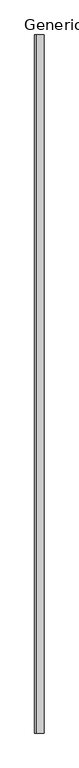
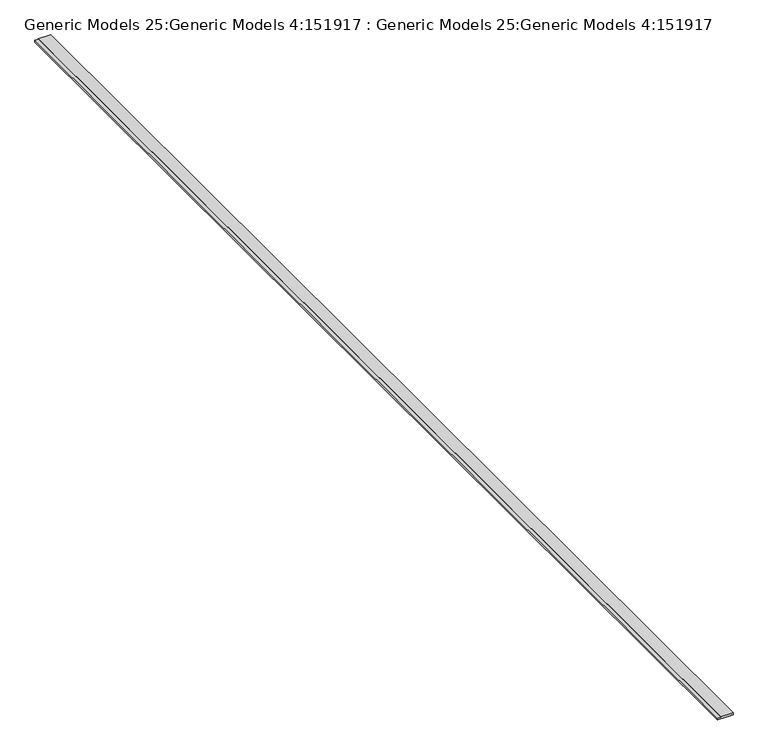
"""IFC4 building model written with IfcOpenShell, lengths in millimetres: proxy geometry, Generic Models 25:Generic Models 4:151917 : Generic Models 25:Generic Models 4:151917."""

from ifc_helpers import new_model, si_unit, frame, origin, place, context, project, spatial, polyline, outline, extrude, source, transform, mapped, element, save


def generic_models_25_generic_models_4_151917_generic_models_25_53bbe27b(model_context):
    return source(origin(), model_context, "Body", "SweptSolid", [
        extrude(outline(polyline([(3046.095, 8497.8650291), (3046.095, 8520.308213), (3067.05, 8520.308213), (3067.05, 8390.926963), (3065.78, 8390.926963), (3065.78, 8354.096963), (3046.095, 8354.096963), (3046.095, 8356.306763), (3047.8274564, 8356.306763), (3047.8274564, 8357.576763), (3044.825, 8357.576763), (3044.825, 8497.8650291), (3046.095, 8497.8650291)])), frame((0.0, -477.1974793, 0.0), z_axis=(0.0, 1.0, 0.0), x_axis=(0.0, 0.0, 1.0)), (0.0, 0.0, 1.0), 12446.0),
    ])


if __name__ == "__main__":
    model = new_model("IFC4")
    model_context = context("Model", 3, world=origin())
    ifc_project = project(units=[si_unit("LENGTHUNIT", "METRE", prefix="MILLI")], contexts=[model_context])
    site = spatial("IfcSite", under=ifc_project)
    building = spatial("IfcBuilding", under=site)
    placement = place(None, origin())
    generic_models_25_generic_models_4_151917_generic_models_25_shape = generic_models_25_generic_models_4_151917_generic_models_25_53bbe27b(model_context)
    element("IfcBuildingElementProxy", 1, Name="Generic Models 25:Generic Models 4:151917 : Generic Models 25:Generic Models 4:151917", ObjectType="Generic Models 25:Generic Models 4:151917 : Generic Models 25:Generic Models 4:151917", at=placement, inside=building, context=model_context, shape_type="MappedRepresentation", body=[
        mapped(generic_models_25_generic_models_4_151917_generic_models_25_shape, transform((0.0, 0.0, 0.0), x_axis=(1.0, 0.0, 0.0), y_axis=(0.0, 1.0, 0.0), z_axis=(0.0, 0.0, 1.0))),
    ])
    save(model, "model.ifc")

# Revit data of these elements
# Type "Generic Models 25:Generic Models 4:151917 : Generic Models 25:Generic Models 4:151917"
#   NameOverride = "Generic Models 25:Generic Models 4:151917"
#   ObjectTypeOverride = "Generic Models 25:Generic Models 4"
#   Reference = "Generic Models 4"
#   Category = "Generic Models"
#   Tag = "151917"
# Element 1 (IfcBuildingElementProxy, "Generic Models 25:Generic Models 4:151917 : Generic Models 25:Generic Models 4:151917")
#   Materials on its faces: "_7/8\" SMOOTH TROWEL EXTERIOR STUCCO (COLOR PER OWNER) 770"
# Materials
#   "_7/8\" SMOOTH TROWEL EXTERIOR STUCCO (COLOR PER OWNER) 770": class "Unassigned", colour RGB 233 233 233, transparency 0
